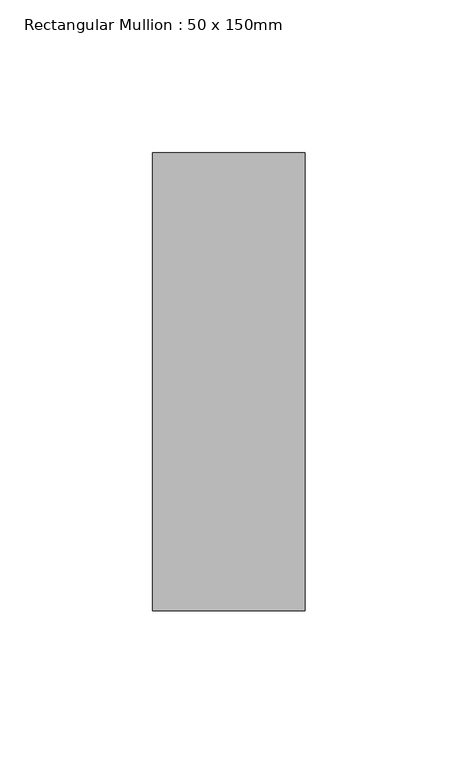
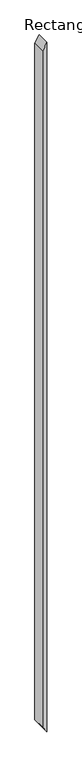
"""IFC4 building model written with IfcOpenShell, lengths in millimetres: member geometry, Rectangular Mullion : 50 x 150mm."""

from ifc_helpers import new_model, si_unit, frame, origin, place, context, project, spatial, polyline, outline, extrude, source, transform, mapped, element, save


def rectangular_mullion_50_x_150mm_6888afb9(model_context):
    return source(origin(), model_context, "Body", "SweptSolid", [
        extrude(outline(polyline([(0.0, 0.0), (-85.321119, -50.0), (-8217.0308307, -50.0), (-8288.6527046, 0.0), (0.0, 0.0)])), frame((0.0, -75.0, 0.0), z_axis=(0.0, 1.0, 0.0), x_axis=(0.0, 0.0, 1.0)), (0.0, 0.0, 1.0), 150.0),
    ])


if __name__ == "__main__":
    model = new_model("IFC4")
    model_context = context("Model", 3, world=origin())
    ifc_project = project(units=[si_unit("LENGTHUNIT", "METRE", prefix="MILLI")], contexts=[model_context])
    site = spatial("IfcSite", under=ifc_project)
    building = spatial("IfcBuilding", under=site)
    placement = place(None, origin())
    rectangular_mullion_50_x_150mm_shape = rectangular_mullion_50_x_150mm_6888afb9(model_context)
    element("IfcMember", 1, ObjectType="Rectangular Mullion : 50 x 150mm", at=placement, inside=building, context=model_context, shape_type="MappedRepresentation", body=[
        mapped(rectangular_mullion_50_x_150mm_shape, transform((0.0, 0.0, 0.0), x_axis=(1.0, 0.0, 0.0), y_axis=(0.0, 1.0, 0.0), z_axis=(0.0, 0.0, 1.0))),
    ])
    save(model, "model.ifc")

# Revit data of these elements
# Type "Rectangular Mullion : 50 x 150mm"
#   built-in parameter 1007304 = 0.492126 (stored number, unit not read)
#   built-in parameter 1007301 = 0.082021 (stored number, unit not read)
#   built-in parameter 1007300 = 0.082021 (stored number, unit not read)
# Element 1 (IfcMember, "Rectangular Mullion : 50 x 150mm")
#   Materials on its faces: "Metal - Aluminium"
# Materials
#   "Metal - Aluminium": class "Metal", colour RGB 247 247 247, transparency 0
